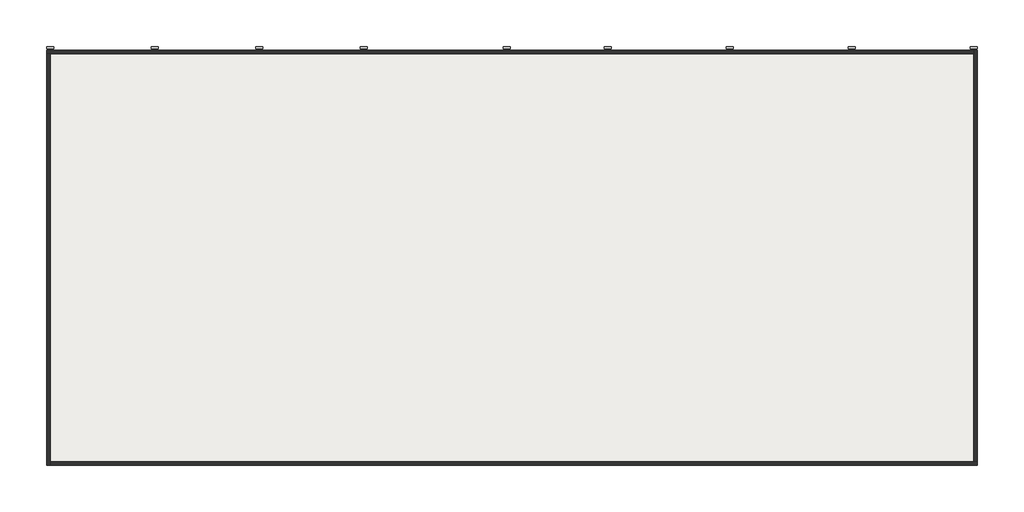
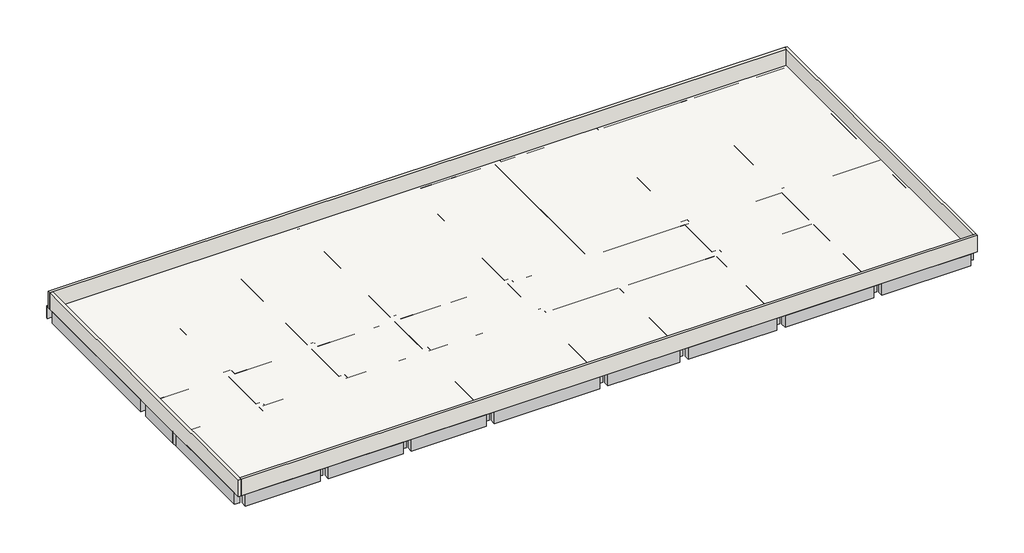
# One storey: 59 beams, 4 walls, 1 slab.
"""IFC4 building model written with IfcOpenShell, lengths in millimetres."""

from ifc_helpers import new_model, si_unit, frame, origin, place, context, project, spatial, polyline, outline, extrude, faceted_brep, element, save

model = new_model("IFC4")

# Units and contexts
model_context = context("Model", 3, world=origin())
ifc_project = project(units=[si_unit("LENGTHUNIT", "METRE", prefix="MILLI")], contexts=[model_context])

# Site, building, storey
site = spatial("IfcSite", under=ifc_project)
building = spatial("IfcBuilding", under=site)
storey = spatial("IfcBuildingStorey", under=building, Name="TOC", Elevation=7650.0)

# Beams
placement = place(None, origin())
element("IfcBeam", 1, ObjectType="RC Beam_Rectangular : H_SB_ACB_B400xH900", at=placement, inside=storey, context=model_context, shape_type="SweptSolid", body=[
    extrude(outline(polyline([(224.7, 12116.5208589), (224.7, 12516.5208589), (5624.7, 12516.5208589), (5624.7, 12116.5208589), (224.7, 12116.5208589)])), frame((0.0, 0.0, 6750.0), z_axis=(0.0, 0.0, 1.0), x_axis=(1.0, 0.0, 0.0)), (0.0, 0.0, 1.0), 900.0),
])
element("IfcBeam", 2, ObjectType="RC Beam_Rectangular : H_SB_ACB_B400xH900", at=placement, inside=storey, context=model_context, shape_type="SweptSolid", body=[
    extrude(outline(polyline([(6224.7, 12116.5208589), (6224.7, 12516.5208589), (11624.7, 12516.5208589), (11624.7, 12116.5208589), (6224.7, 12116.5208589)])), frame((0.0, 0.0, 6750.0), z_axis=(0.0, 0.0, 1.0), x_axis=(1.0, 0.0, 0.0)), (0.0, 0.0, 1.0), 900.0),
])
element("IfcBeam", 3, ObjectType="RC Beam_Rectangular : H_SB_ACB_B400xH900", at=placement, inside=storey, context=model_context, shape_type="SweptSolid", body=[
    extrude(outline(polyline([(12224.7, 12116.5208589), (12224.7, 12516.5208589), (17624.7, 12516.5208589), (17624.7, 12116.5208589), (12224.7, 12116.5208589)])), frame((0.0, 0.0, 6750.0), z_axis=(0.0, 0.0, 1.0), x_axis=(1.0, 0.0, 0.0)), (0.0, 0.0, 1.0), 900.0),
])
element("IfcBeam", 4, ObjectType="RC Beam_Rectangular : H_SB_ACB_B400xH900", at=placement, inside=storey, context=model_context, shape_type="Brep", body=[
    faceted_brep([(26324.7, 12116.5208589, 7650.0), (26324.7, 12516.5208589, 7650.0), (25924.7, 12516.5208589, 7650.0), (18224.7, 12516.5208589, 7650.0), (18224.7, 12116.5208589, 7650.0), (25924.7, 12116.5208589, 7650.0), (26324.7, 12116.5208589, 6750.0), (18224.7, 12116.5208589, 6750.0), (25924.7, 12116.5208589, 6750.0), (26324.7, 12516.5208589, 6750.0), (18224.7, 12516.5208589, 6750.0), (25924.7, 12516.5208589, 6750.0)], [[[0, 1, 2, 3, 4, 5]], [[6, 0, 5, 4, 7, 8]], [[9, 6, 8, 7, 10, 11]], [[1, 9, 11, 10, 3, 2]], [[4, 3, 10, 7]], [[1, 0, 6, 9]]]),
])
element("IfcBeam", 5, ObjectType="RC Beam_Rectangular : H_SB_ACB_B400xH900", at=placement, inside=storey, context=model_context, shape_type="Brep", body=[
    faceted_brep([(32124.7, 12116.5208589, 7650.0), (32124.7, 12516.5208589, 7650.0), (31724.7, 12516.5208589, 7650.0), (26324.7, 12516.5208589, 7650.0), (26324.7, 12116.5208589, 7650.0), (31724.7, 12116.5208589, 7650.0), (32124.7, 12116.5208589, 6750.0), (26324.7, 12116.5208589, 6750.0), (31724.7, 12116.5208589, 6750.0), (32124.7, 12516.5208589, 6750.0), (26324.7, 12516.5208589, 6750.0), (31724.7, 12516.5208589, 6750.0)], [[[0, 1, 2, 3, 4, 5]], [[6, 0, 5, 4, 7, 8]], [[9, 6, 8, 7, 10, 11]], [[1, 9, 11, 10, 3, 2]], [[1, 0, 6, 9]], [[4, 3, 10, 7]]]),
])
element("IfcBeam", 6, ObjectType="RC Beam_Rectangular : H_SB_ACB_B400xH900", at=placement, inside=storey, context=model_context, shape_type="Brep", body=[
    faceted_brep([(39124.7, 12116.5208589, 7650.0), (39124.7, 12516.5208589, 7650.0), (38724.7, 12516.5208589, 7650.0), (32124.7, 12516.5208589, 7650.0), (32124.7, 12116.5208589, 7650.0), (38724.7, 12116.5208589, 7650.0), (39124.7, 12116.5208589, 6750.0), (32124.7, 12116.5208589, 6750.0), (38724.7, 12116.5208589, 6750.0), (39124.7, 12516.5208589, 6750.0), (32124.7, 12516.5208589, 6750.0), (38724.7, 12516.5208589, 6750.0)], [[[0, 1, 2, 3, 4, 5]], [[6, 0, 5, 4, 7, 8]], [[9, 6, 8, 7, 10, 11]], [[1, 9, 11, 10, 3, 2]], [[1, 0, 6, 9]], [[4, 3, 10, 7]]]),
])
element("IfcBeam", 7, ObjectType="RC Beam_Rectangular : H_SB_ACB_B400xH900", at=placement, inside=storey, context=model_context, shape_type="Brep", body=[
    faceted_brep([(46124.7, 12116.5208589, 7650.0), (46124.7, 12516.5208589, 7650.0), (45724.7, 12516.5208589, 7650.0), (39124.7, 12516.5208589, 7650.0), (39124.7, 12116.5208589, 7650.0), (45724.7, 12116.5208589, 7650.0), (46124.7, 12116.5208589, 6750.0), (39124.7, 12116.5208589, 6750.0), (45724.7, 12116.5208589, 6750.0), (46124.7, 12516.5208589, 6750.0), (39124.7, 12516.5208589, 6750.0), (45724.7, 12516.5208589, 6750.0)], [[[0, 1, 2, 3, 4, 5]], [[6, 0, 5, 4, 7, 8]], [[9, 6, 8, 7, 10, 11]], [[1, 9, 11, 10, 3, 2]], [[1, 0, 6, 9]], [[4, 3, 10, 7]]]),
])
element("IfcBeam", 8, ObjectType="RC Beam_Rectangular : H_SB_ACB_B400xH900", at=placement, inside=storey, context=model_context, shape_type="Brep", body=[
    faceted_brep([(53124.7, 12116.5208589, 7650.0), (53124.7, 12516.5208589, 7650.0), (52724.7, 12516.5208589, 7650.0), (46124.7, 12516.5208589, 7650.0), (46124.7, 12116.5208589, 7650.0), (52724.7, 12116.5208589, 7650.0), (53124.7, 12116.5208589, 6750.0), (46124.7, 12116.5208589, 6750.0), (52724.7, 12116.5208589, 6750.0), (53124.7, 12516.5208589, 6750.0), (46124.7, 12516.5208589, 6750.0), (52724.7, 12516.5208589, 6750.0)], [[[0, 1, 2, 3, 4, 5]], [[6, 0, 5, 4, 7, 8]], [[9, 6, 8, 7, 10, 11]], [[1, 9, 11, 10, 3, 2]], [[1, 0, 6, 9]], [[4, 3, 10, 7]]]),
])
element("IfcBeam", 9, ObjectType="RC Beam_Rectangular : H_SB_ACB_B400xH900", at=placement, inside=storey, context=model_context, shape_type="SweptSolid", body=[
    extrude(outline(polyline([(224.7, 23816.5208589), (224.7, 24216.5208589), (5624.7, 24216.5208589), (5624.7, 23816.5208589), (224.7, 23816.5208589)])), frame((0.0, 0.0, 6750.0), z_axis=(0.0, 0.0, 1.0), x_axis=(1.0, 0.0, 0.0)), (0.0, 0.0, 1.0), 900.0),
])
element("IfcBeam", 10, ObjectType="RC Beam_Rectangular : H_SB_ACB_B400xH900", at=placement, inside=storey, context=model_context, shape_type="SweptSolid", body=[
    extrude(outline(polyline([(6224.7, 23816.5208589), (6224.7, 24216.5208589), (11624.7, 24216.5208589), (11624.7, 23816.5208589), (6224.7, 23816.5208589)])), frame((0.0, 0.0, 6750.0), z_axis=(0.0, 0.0, 1.0), x_axis=(1.0, 0.0, 0.0)), (0.0, 0.0, 1.0), 900.0),
])
element("IfcBeam", 11, ObjectType="RC Beam_Rectangular : H_SB_ACB_B400xH900", at=placement, inside=storey, context=model_context, shape_type="SweptSolid", body=[
    extrude(outline(polyline([(12224.7, 23816.5208589), (12224.7, 24216.5208589), (17624.7, 24216.5208589), (17624.7, 23816.5208589), (12224.7, 23816.5208589)])), frame((0.0, 0.0, 6750.0), z_axis=(0.0, 0.0, 1.0), x_axis=(1.0, 0.0, 0.0)), (0.0, 0.0, 1.0), 900.0),
])
element("IfcBeam", 12, ObjectType="RC Beam_Rectangular : H_SB_ACB_B400xH900", at=placement, inside=storey, context=model_context, shape_type="SweptSolid", body=[
    extrude(outline(polyline([(18224.7, 23816.5208589), (18224.7, 24216.5208589), (25824.7, 24216.5208589), (25824.7, 23816.5208589), (18224.7, 23816.5208589)])), frame((0.0, 0.0, 6750.0), z_axis=(0.0, 0.0, 1.0), x_axis=(1.0, 0.0, 0.0)), (0.0, 0.0, 1.0), 900.0),
])
element("IfcBeam", 13, ObjectType="RC Beam_Rectangular : H_SB_ACB_B400xH900", at=placement, inside=storey, context=model_context, shape_type="SweptSolid", body=[
    extrude(outline(polyline([(26424.7, 23816.5208589), (26424.7, 24216.5208589), (31624.7, 24216.5208589), (31624.7, 23816.5208589), (26424.7, 23816.5208589)])), frame((0.0, 0.0, 6750.0), z_axis=(0.0, 0.0, 1.0), x_axis=(1.0, 0.0, 0.0)), (0.0, 0.0, 1.0), 900.0),
])
element("IfcBeam", 14, ObjectType="RC Beam_Rectangular : H_SB_ACB_B400xH900", at=placement, inside=storey, context=model_context, shape_type="SweptSolid", body=[
    extrude(outline(polyline([(32224.7, 23816.5208589), (32224.7, 24216.5208589), (38624.7, 24216.5208589), (38624.7, 23816.5208589), (32224.7, 23816.5208589)])), frame((0.0, 0.0, 6750.0), z_axis=(0.0, 0.0, 1.0), x_axis=(1.0, 0.0, 0.0)), (0.0, 0.0, 1.0), 900.0),
])
element("IfcBeam", 15, ObjectType="RC Beam_Rectangular : H_SB_ACB_B400xH900", at=placement, inside=storey, context=model_context, shape_type="SweptSolid", body=[
    extrude(outline(polyline([(39224.7, 23816.5208589), (39224.7, 24216.5208589), (45624.7, 24216.5208589), (45624.7, 23816.5208589), (39224.7, 23816.5208589)])), frame((0.0, 0.0, 6750.0), z_axis=(0.0, 0.0, 1.0), x_axis=(1.0, 0.0, 0.0)), (0.0, 0.0, 1.0), 900.0),
])
element("IfcBeam", 16, ObjectType="RC Beam_Rectangular : H_SB_ACB_B400xH900", at=placement, inside=storey, context=model_context, shape_type="SweptSolid", body=[
    extrude(outline(polyline([(46224.7, 23816.5208589), (46224.7, 24216.5208589), (52624.7, 24216.5208589), (52624.7, 23816.5208589), (46224.7, 23816.5208589)])), frame((0.0, 0.0, 6750.0), z_axis=(0.0, 0.0, 1.0), x_axis=(1.0, 0.0, 0.0)), (0.0, 0.0, 1.0), 900.0),
])
element("IfcBeam", 17, ObjectType="RC Beam_Rectangular : H_SB_ACB_B400xH900", at=placement, inside=storey, context=model_context, shape_type="Brep", body=[
    faceted_brep([(-275.3, 8616.5208589, 7650.0), (-275.3, 8216.5208589, 7650.0), (124.7, 8216.5208589, 7650.0), (5724.7, 8216.5208589, 7650.0), (6124.7, 8216.5208589, 7650.0), (6124.7, 8616.5208589, 7650.0), (5724.7, 8616.5208589, 7650.0), (124.7, 8616.5208589, 7650.0), (-275.3, 8216.5208589, 6750.0), (124.7, 8216.5208589, 6750.0), (5724.7, 8216.5208589, 6750.0), (6124.7, 8216.5208589, 6750.0), (-275.3, 8616.5208589, 6750.0), (124.7, 8616.5208589, 6750.0), (5724.7, 8616.5208589, 6750.0), (6124.7, 8616.5208589, 6750.0)], [[[0, 1, 2, 3, 4, 5, 6, 7]], [[1, 8, 9, 10, 11, 4, 3, 2]], [[8, 12, 13, 14, 15, 11, 10, 9]], [[12, 0, 7, 6, 5, 15, 14, 13]], [[1, 0, 12, 8]], [[5, 4, 11, 15]]]),
])
element("IfcBeam", 18, ObjectType="RC Beam_Rectangular : H_SB_ACB_B400xH900", at=placement, inside=storey, context=model_context, shape_type="Brep", body=[
    faceted_brep([(12124.7, 8216.5208589, 7650.0), (12124.7, 8616.5208589, 7650.0), (11724.7, 8616.5208589, 7650.0), (6124.7, 8616.5208589, 7650.0), (6124.7, 8216.5208589, 7650.0), (11724.7, 8216.5208589, 7650.0), (12124.7, 8216.5208589, 6750.0), (6124.7, 8216.5208589, 6750.0), (11724.7, 8216.5208589, 6750.0), (12124.7, 8616.5208589, 6750.0), (6124.7, 8616.5208589, 6750.0), (11724.7, 8616.5208589, 6750.0)], [[[0, 1, 2, 3, 4, 5]], [[6, 0, 5, 4, 7, 8]], [[9, 6, 8, 7, 10, 11]], [[1, 9, 11, 10, 3, 2]], [[1, 0, 6, 9]], [[4, 3, 10, 7]]]),
])
element("IfcBeam", 19, ObjectType="RC Beam_Rectangular : H_SB_ACB_B400xH900", at=placement, inside=storey, context=model_context, shape_type="Brep", body=[
    faceted_brep([(18124.7, 8216.5208589, 7650.0), (18124.7, 8616.5208589, 7650.0), (17724.7, 8616.5208589, 7650.0), (12124.7, 8616.5208589, 7650.0), (12124.7, 8216.5208589, 7650.0), (17724.7, 8216.5208589, 7650.0), (18124.7, 8216.5208589, 6750.0), (12124.7, 8216.5208589, 6750.0), (17724.7, 8216.5208589, 6750.0), (18124.7, 8616.5208589, 6750.0), (12124.7, 8616.5208589, 6750.0), (17724.7, 8616.5208589, 6750.0)], [[[0, 1, 2, 3, 4, 5]], [[6, 0, 5, 4, 7, 8]], [[9, 6, 8, 7, 10, 11]], [[1, 9, 11, 10, 3, 2]], [[1, 0, 6, 9]], [[4, 3, 10, 7]]]),
])
element("IfcBeam", 20, ObjectType="RC Beam_Rectangular : H_SB_ACB_B400xH900", at=placement, inside=storey, context=model_context, shape_type="SweptSolid", body=[
    extrude(outline(polyline([(18124.7, 8216.5208589), (18124.7, 8616.5208589), (25824.7, 8616.5208589), (25824.7, 8216.5208589), (18124.7, 8216.5208589)])), frame((0.0, 0.0, 6750.0), z_axis=(0.0, 0.0, 1.0), x_axis=(1.0, 0.0, 0.0)), (0.0, 0.0, 1.0), 900.0),
])
element("IfcBeam", 21, ObjectType="RC Beam_Rectangular : H_SB_ACB_B400xH900", at=placement, inside=storey, context=model_context, shape_type="SweptSolid", body=[
    extrude(outline(polyline([(26424.7, 8216.5208589), (26424.7, 8616.5208589), (31624.7, 8616.5208589), (31624.7, 8216.5208589), (26424.7, 8216.5208589)])), frame((0.0, 0.0, 6750.0), z_axis=(0.0, 0.0, 1.0), x_axis=(1.0, 0.0, 0.0)), (0.0, 0.0, 1.0), 900.0),
])
element("IfcBeam", 22, ObjectType="RC Beam_Rectangular : H_SB_ACB_B400xH900", at=placement, inside=storey, context=model_context, shape_type="SweptSolid", body=[
    extrude(outline(polyline([(32224.7, 8216.5208589), (32224.7, 8616.5208589), (38624.7, 8616.5208589), (38624.7, 8216.5208589), (32224.7, 8216.5208589)])), frame((0.0, 0.0, 6750.0), z_axis=(0.0, 0.0, 1.0), x_axis=(1.0, 0.0, 0.0)), (0.0, 0.0, 1.0), 900.0),
])
element("IfcBeam", 23, ObjectType="RC Beam_Rectangular : H_SB_ACB_B400xH900", at=placement, inside=storey, context=model_context, shape_type="SweptSolid", body=[
    extrude(outline(polyline([(39224.7, 8216.5208589), (39224.7, 8616.5208589), (45624.7, 8616.5208589), (45624.7, 8216.5208589), (39224.7, 8216.5208589)])), frame((0.0, 0.0, 6750.0), z_axis=(0.0, 0.0, 1.0), x_axis=(1.0, 0.0, 0.0)), (0.0, 0.0, 1.0), 900.0),
])
element("IfcBeam", 24, ObjectType="RC Beam_Rectangular : H_SB_ACB_B400xH900", at=placement, inside=storey, context=model_context, shape_type="SweptSolid", body=[
    extrude(outline(polyline([(46224.7, 8216.5208589), (46224.7, 8616.5208589), (52624.7, 8616.5208589), (52624.7, 8216.5208589), (46224.7, 8216.5208589)])), frame((0.0, 0.0, 6750.0), z_axis=(0.0, 0.0, 1.0), x_axis=(1.0, 0.0, 0.0)), (0.0, 0.0, 1.0), 900.0),
])
element("IfcBeam", 25, ObjectType="RC Beam_Rectangular : H_SB_ACB_B400xH900", at=placement, inside=storey, context=model_context, shape_type="SweptSolid", body=[
    extrude(outline(polyline([(224.7, 416.5208589), (224.7, 816.5208589), (5624.7, 816.5208589), (5624.7, 416.5208589), (224.7, 416.5208589)])), frame((0.0, 0.0, 6750.0), z_axis=(0.0, 0.0, 1.0), x_axis=(1.0, 0.0, 0.0)), (0.0, 0.0, 1.0), 900.0),
])
element("IfcBeam", 26, ObjectType="RC Beam_Rectangular : H_SB_ACB_B400xH900", at=placement, inside=storey, context=model_context, shape_type="SweptSolid", body=[
    extrude(outline(polyline([(6224.7, 416.5208589), (6224.7, 816.5208589), (11624.7, 816.5208589), (11624.7, 416.5208589), (6224.7, 416.5208589)])), frame((0.0, 0.0, 6750.0), z_axis=(0.0, 0.0, 1.0), x_axis=(1.0, 0.0, 0.0)), (0.0, 0.0, 1.0), 900.0),
])
element("IfcBeam", 27, ObjectType="RC Beam_Rectangular : H_SB_ACB_B400xH900", at=placement, inside=storey, context=model_context, shape_type="SweptSolid", body=[
    extrude(outline(polyline([(12224.7, 416.5208589), (12224.7, 816.5208589), (17624.7, 816.5208589), (17624.7, 416.5208589), (12224.7, 416.5208589)])), frame((0.0, 0.0, 6750.0), z_axis=(0.0, 0.0, 1.0), x_axis=(1.0, 0.0, 0.0)), (0.0, 0.0, 1.0), 900.0),
])
element("IfcBeam", 28, ObjectType="RC Beam_Rectangular : H_SB_ACB_B400xH900", at=placement, inside=storey, context=model_context, shape_type="SweptSolid", body=[
    extrude(outline(polyline([(18224.7, 416.5208589), (18224.7, 816.5208589), (25824.7, 816.5208589), (25824.7, 416.5208589), (18224.7, 416.5208589)])), frame((0.0, 0.0, 6750.0), z_axis=(0.0, 0.0, 1.0), x_axis=(1.0, 0.0, 0.0)), (0.0, 0.0, 1.0), 900.0),
])
element("IfcBeam", 29, ObjectType="RC Beam_Rectangular : H_SB_ACB_B400xH900", at=placement, inside=storey, context=model_context, shape_type="SweptSolid", body=[
    extrude(outline(polyline([(26424.7, 416.5208589), (26424.7, 816.5208589), (31624.7, 816.5208589), (31624.7, 416.5208589), (26424.7, 416.5208589)])), frame((0.0, 0.0, 6750.0), z_axis=(0.0, 0.0, 1.0), x_axis=(1.0, 0.0, 0.0)), (0.0, 0.0, 1.0), 900.0),
])
element("IfcBeam", 30, ObjectType="RC Beam_Rectangular : H_SB_ACB_B400xH900", at=placement, inside=storey, context=model_context, shape_type="SweptSolid", body=[
    extrude(outline(polyline([(32224.7, 416.5208589), (32224.7, 816.5208589), (38624.7, 816.5208589), (38624.7, 416.5208589), (32224.7, 416.5208589)])), frame((0.0, 0.0, 6750.0), z_axis=(0.0, 0.0, 1.0), x_axis=(1.0, 0.0, 0.0)), (0.0, 0.0, 1.0), 900.0),
])
element("IfcBeam", 31, ObjectType="RC Beam_Rectangular : H_SB_ACB_B400xH900", at=placement, inside=storey, context=model_context, shape_type="SweptSolid", body=[
    extrude(outline(polyline([(39224.7, 416.5208589), (39224.7, 816.5208589), (45624.7, 816.5208589), (45624.7, 416.5208589), (39224.7, 416.5208589)])), frame((0.0, 0.0, 6750.0), z_axis=(0.0, 0.0, 1.0), x_axis=(1.0, 0.0, 0.0)), (0.0, 0.0, 1.0), 900.0),
])
element("IfcBeam", 32, ObjectType="RC Beam_Rectangular : H_SB_ACB_B400xH900", at=placement, inside=storey, context=model_context, shape_type="SweptSolid", body=[
    extrude(outline(polyline([(46224.7, 416.5208589), (46224.7, 816.5208589), (52624.7, 816.5208589), (52624.7, 416.5208589), (46224.7, 416.5208589)])), frame((0.0, 0.0, 6750.0), z_axis=(0.0, 0.0, 1.0), x_axis=(1.0, 0.0, 0.0)), (0.0, 0.0, 1.0), 900.0),
])
element("IfcBeam", 33, ObjectType="RC Beam_Rectangular : H_SB_ACB_B400xH900", at=placement, inside=storey, context=model_context, shape_type="SweptSolid", body=[
    extrude(outline(polyline([(-275.3, 8216.5208589), (124.7, 8216.5208589), (124.7, 916.5208589), (-275.3, 916.5208589), (-275.3, 8216.5208589)])), frame((0.0, 0.0, 6750.0), z_axis=(0.0, 0.0, 1.0), x_axis=(1.0, 0.0, 0.0)), (0.0, 0.0, 1.0), 900.0),
])
element("IfcBeam", 34, ObjectType="RC Beam_Rectangular : H_SB_ACB_B400xH900", at=placement, inside=storey, context=model_context, shape_type="SweptSolid", body=[
    extrude(outline(polyline([(124.7, 8616.5208589), (-275.3, 8616.5208589), (-275.3, 12016.5208589), (124.7, 12016.5208589), (124.7, 8616.5208589)])), frame((0.0, 0.0, 6750.0), z_axis=(0.0, 0.0, 1.0), x_axis=(1.0, 0.0, 0.0)), (0.0, 0.0, 1.0), 900.0),
])
element("IfcBeam", 35, ObjectType="RC Beam_Rectangular : H_SB_ACB_B400xH900", at=placement, inside=storey, context=model_context, shape_type="SweptSolid", body=[
    extrude(outline(polyline([(-275.3, 24429.2208589), (124.7, 24429.2208589), (124.7, 24316.5208589), (-275.3, 24316.5208589), (-275.3, 24429.2208589)])), frame((0.0, 0.0, 6750.0), z_axis=(0.0, 0.0, 1.0), x_axis=(1.0, 0.0, 0.0)), (0.0, 0.0, 1.0), 900.0),
    extrude(outline(polyline([(124.7, 12616.5208589), (-275.3, 12616.5208589), (-275.3, 23716.5208589), (124.7, 23716.5208589), (124.7, 12616.5208589)])), frame((0.0, 0.0, 6750.0), z_axis=(0.0, 0.0, 1.0), x_axis=(1.0, 0.0, 0.0)), (0.0, 0.0, 1.0), 900.0),
])
element("IfcBeam", 36, ObjectType="RC Beam_Rectangular : H_SB_ACB_B400xH900", at=placement, inside=storey, context=model_context, shape_type="SweptSolid", body=[
    extrude(outline(polyline([(5724.7, 8216.5208589), (6124.7, 8216.5208589), (6124.7, 916.5208589), (5724.7, 916.5208589), (5724.7, 8216.5208589)])), frame((0.0, 0.0, 6750.0), z_axis=(0.0, 0.0, 1.0), x_axis=(1.0, 0.0, 0.0)), (0.0, 0.0, 1.0), 900.0),
])
element("IfcBeam", 37, ObjectType="RC Beam_Rectangular : H_SB_ACB_B400xH900", at=placement, inside=storey, context=model_context, shape_type="SweptSolid", body=[
    extrude(outline(polyline([(6124.7, 8616.5208589), (5724.7, 8616.5208589), (5724.7, 12016.5208589), (6124.7, 12016.5208589), (6124.7, 8616.5208589)])), frame((0.0, 0.0, 6750.0), z_axis=(0.0, 0.0, 1.0), x_axis=(1.0, 0.0, 0.0)), (0.0, 0.0, 1.0), 900.0),
])
element("IfcBeam", 38, ObjectType="RC Beam_Rectangular : H_SB_ACB_B400xH900", at=placement, inside=storey, context=model_context, shape_type="SweptSolid", body=[
    extrude(outline(polyline([(5724.7, 24429.2208589), (6124.7, 24429.2208589), (6124.7, 24316.5208589), (5724.7, 24316.5208589), (5724.7, 24429.2208589)])), frame((0.0, 0.0, 6750.0), z_axis=(0.0, 0.0, 1.0), x_axis=(1.0, 0.0, 0.0)), (0.0, 0.0, 1.0), 900.0),
    extrude(outline(polyline([(6124.7, 12616.5208589), (5724.7, 12616.5208589), (5724.7, 23716.5208589), (6124.7, 23716.5208589), (6124.7, 12616.5208589)])), frame((0.0, 0.0, 6750.0), z_axis=(0.0, 0.0, 1.0), x_axis=(1.0, 0.0, 0.0)), (0.0, 0.0, 1.0), 900.0),
])
element("IfcBeam", 39, ObjectType="RC Beam_Rectangular : H_SB_ACB_B400xH900", at=placement, inside=storey, context=model_context, shape_type="SweptSolid", body=[
    extrude(outline(polyline([(11724.7, 8216.5208589), (12124.7, 8216.5208589), (12124.7, 916.5208589), (11724.7, 916.5208589), (11724.7, 8216.5208589)])), frame((0.0, 0.0, 6750.0), z_axis=(0.0, 0.0, 1.0), x_axis=(1.0, 0.0, 0.0)), (0.0, 0.0, 1.0), 900.0),
])
element("IfcBeam", 40, ObjectType="RC Beam_Rectangular : H_SB_ACB_B400xH900", at=placement, inside=storey, context=model_context, shape_type="SweptSolid", body=[
    extrude(outline(polyline([(12124.7, 8616.5208589), (11724.7, 8616.5208589), (11724.7, 12016.5208589), (12124.7, 12016.5208589), (12124.7, 8616.5208589)])), frame((0.0, 0.0, 6750.0), z_axis=(0.0, 0.0, 1.0), x_axis=(1.0, 0.0, 0.0)), (0.0, 0.0, 1.0), 900.0),
])
element("IfcBeam", 41, ObjectType="RC Beam_Rectangular : H_SB_ACB_B400xH900", at=placement, inside=storey, context=model_context, shape_type="SweptSolid", body=[
    extrude(outline(polyline([(11724.7, 24429.2208589), (12124.7, 24429.2208589), (12124.7, 24316.5208589), (11724.7, 24316.5208589), (11724.7, 24429.2208589)])), frame((0.0, 0.0, 6750.0), z_axis=(0.0, 0.0, 1.0), x_axis=(1.0, 0.0, 0.0)), (0.0, 0.0, 1.0), 900.0),
    extrude(outline(polyline([(12124.7, 12616.5208589), (11724.7, 12616.5208589), (11724.7, 23716.5208589), (12124.7, 23716.5208589), (12124.7, 12616.5208589)])), frame((0.0, 0.0, 6750.0), z_axis=(0.0, 0.0, 1.0), x_axis=(1.0, 0.0, 0.0)), (0.0, 0.0, 1.0), 900.0),
])
element("IfcBeam", 42, ObjectType="RC Beam_Rectangular : H_SB_ACB_B400xH900", at=placement, inside=storey, context=model_context, shape_type="SweptSolid", body=[
    extrude(outline(polyline([(17724.7, 8216.5208589), (18124.7, 8216.5208589), (18124.7, 916.5208589), (17724.7, 916.5208589), (17724.7, 8216.5208589)])), frame((0.0, 0.0, 6750.0), z_axis=(0.0, 0.0, 1.0), x_axis=(1.0, 0.0, 0.0)), (0.0, 0.0, 1.0), 900.0),
])
element("IfcBeam", 43, ObjectType="RC Beam_Rectangular : H_SB_ACB_B400xH900", at=placement, inside=storey, context=model_context, shape_type="SweptSolid", body=[
    extrude(outline(polyline([(18124.7, 8616.5208589), (17724.7, 8616.5208589), (17724.7, 12016.5208589), (18124.7, 12016.5208589), (18124.7, 8616.5208589)])), frame((0.0, 0.0, 6750.0), z_axis=(0.0, 0.0, 1.0), x_axis=(1.0, 0.0, 0.0)), (0.0, 0.0, 1.0), 900.0),
])
element("IfcBeam", 44, ObjectType="RC Beam_Rectangular : H_SB_ACB_B400xH900", at=placement, inside=storey, context=model_context, shape_type="SweptSolid", body=[
    extrude(outline(polyline([(17724.7, 24429.2208589), (18124.7, 24429.2208589), (18124.7, 24316.5208589), (17724.7, 24316.5208589), (17724.7, 24429.2208589)])), frame((0.0, 0.0, 6750.0), z_axis=(0.0, 0.0, 1.0), x_axis=(1.0, 0.0, 0.0)), (0.0, 0.0, 1.0), 900.0),
    extrude(outline(polyline([(18124.7, 12616.5208589), (17724.7, 12616.5208589), (17724.7, 23716.5208589), (18124.7, 23716.5208589), (18124.7, 12616.5208589)])), frame((0.0, 0.0, 6750.0), z_axis=(0.0, 0.0, 1.0), x_axis=(1.0, 0.0, 0.0)), (0.0, 0.0, 1.0), 900.0),
])
element("IfcBeam", 45, ObjectType="RC Beam_Rectangular : H_SB_ACB_B400xH900", at=placement, inside=storey, context=model_context, shape_type="SweptSolid", body=[
    extrude(outline(polyline([(25924.7, 8116.5208589), (26324.7, 8116.5208589), (26324.7, 916.5208589), (25924.7, 916.5208589), (25924.7, 8116.5208589)])), frame((0.0, 0.0, 6750.0), z_axis=(0.0, 0.0, 1.0), x_axis=(1.0, 0.0, 0.0)), (0.0, 0.0, 1.0), 900.0),
])
element("IfcBeam", 46, ObjectType="RC Beam_Rectangular : H_SB_ACB_B400xH900", at=placement, inside=storey, context=model_context, shape_type="SweptSolid", body=[
    extrude(outline(polyline([(25924.7, 12116.5208589), (26324.7, 12116.5208589), (26324.7, 8716.5208589), (25924.7, 8716.5208589), (25924.7, 12116.5208589)])), frame((0.0, 0.0, 6750.0), z_axis=(0.0, 0.0, 1.0), x_axis=(1.0, 0.0, 0.0)), (0.0, 0.0, 1.0), 900.0),
])
element("IfcBeam", 47, ObjectType="RC Beam_Rectangular : H_SB_ACB_B400xH900", at=placement, inside=storey, context=model_context, shape_type="SweptSolid", body=[
    extrude(outline(polyline([(25924.7, 24429.2208589), (26324.7, 24429.2208589), (26324.7, 24316.5208589), (25924.7, 24316.5208589), (25924.7, 24429.2208589)])), frame((0.0, 0.0, 6750.0), z_axis=(0.0, 0.0, 1.0), x_axis=(1.0, 0.0, 0.0)), (0.0, 0.0, 1.0), 900.0),
    extrude(outline(polyline([(26324.7, 12516.5208589), (25924.7, 12516.5208589), (25924.7, 23716.5208589), (26324.7, 23716.5208589), (26324.7, 12516.5208589)])), frame((0.0, 0.0, 6750.0), z_axis=(0.0, 0.0, 1.0), x_axis=(1.0, 0.0, 0.0)), (0.0, 0.0, 1.0), 900.0),
])
element("IfcBeam", 48, ObjectType="RC Beam_Rectangular : H_SB_ACB_B400xH900", at=placement, inside=storey, context=model_context, shape_type="SweptSolid", body=[
    extrude(outline(polyline([(31724.7, 8116.5208589), (32124.7, 8116.5208589), (32124.7, 916.5208589), (31724.7, 916.5208589), (31724.7, 8116.5208589)])), frame((0.0, 0.0, 6750.0), z_axis=(0.0, 0.0, 1.0), x_axis=(1.0, 0.0, 0.0)), (0.0, 0.0, 1.0), 900.0),
])
element("IfcBeam", 49, ObjectType="RC Beam_Rectangular : H_SB_ACB_B400xH900", at=placement, inside=storey, context=model_context, shape_type="SweptSolid", body=[
    extrude(outline(polyline([(31724.7, 12116.5208589), (32124.7, 12116.5208589), (32124.7, 8716.5208589), (31724.7, 8716.5208589), (31724.7, 12116.5208589)])), frame((0.0, 0.0, 6750.0), z_axis=(0.0, 0.0, 1.0), x_axis=(1.0, 0.0, 0.0)), (0.0, 0.0, 1.0), 900.0),
])
element("IfcBeam", 50, ObjectType="RC Beam_Rectangular : H_SB_ACB_B400xH900", at=placement, inside=storey, context=model_context, shape_type="SweptSolid", body=[
    extrude(outline(polyline([(31724.7, 24429.2208589), (32124.7, 24429.2208589), (32124.7, 24316.5208589), (31724.7, 24316.5208589), (31724.7, 24429.2208589)])), frame((0.0, 0.0, 6750.0), z_axis=(0.0, 0.0, 1.0), x_axis=(1.0, 0.0, 0.0)), (0.0, 0.0, 1.0), 900.0),
    extrude(outline(polyline([(32124.7, 12516.5208589), (31724.7, 12516.5208589), (31724.7, 23716.5208589), (32124.7, 23716.5208589), (32124.7, 12516.5208589)])), frame((0.0, 0.0, 6750.0), z_axis=(0.0, 0.0, 1.0), x_axis=(1.0, 0.0, 0.0)), (0.0, 0.0, 1.0), 900.0),
])
element("IfcBeam", 51, ObjectType="RC Beam_Rectangular : H_SB_ACB_B400xH900", at=placement, inside=storey, context=model_context, shape_type="SweptSolid", body=[
    extrude(outline(polyline([(38724.7, 8116.5208589), (39124.7, 8116.5208589), (39124.7, 916.5208589), (38724.7, 916.5208589), (38724.7, 8116.5208589)])), frame((0.0, 0.0, 6750.0), z_axis=(0.0, 0.0, 1.0), x_axis=(1.0, 0.0, 0.0)), (0.0, 0.0, 1.0), 900.0),
])
element("IfcBeam", 52, ObjectType="RC Beam_Rectangular : H_SB_ACB_B400xH900", at=placement, inside=storey, context=model_context, shape_type="SweptSolid", body=[
    extrude(outline(polyline([(38724.7, 12116.5208589), (39124.7, 12116.5208589), (39124.7, 8716.5208589), (38724.7, 8716.5208589), (38724.7, 12116.5208589)])), frame((0.0, 0.0, 6750.0), z_axis=(0.0, 0.0, 1.0), x_axis=(1.0, 0.0, 0.0)), (0.0, 0.0, 1.0), 900.0),
])
element("IfcBeam", 53, ObjectType="RC Beam_Rectangular : H_SB_ACB_B400xH900", at=placement, inside=storey, context=model_context, shape_type="SweptSolid", body=[
    extrude(outline(polyline([(38724.7, 24429.2208589), (39124.7, 24429.2208589), (39124.7, 24316.5208589), (38724.7, 24316.5208589), (38724.7, 24429.2208589)])), frame((0.0, 0.0, 6750.0), z_axis=(0.0, 0.0, 1.0), x_axis=(1.0, 0.0, 0.0)), (0.0, 0.0, 1.0), 900.0),
    extrude(outline(polyline([(39124.7, 12516.5208589), (38724.7, 12516.5208589), (38724.7, 23716.5208589), (39124.7, 23716.5208589), (39124.7, 12516.5208589)])), frame((0.0, 0.0, 6750.0), z_axis=(0.0, 0.0, 1.0), x_axis=(1.0, 0.0, 0.0)), (0.0, 0.0, 1.0), 900.0),
])
element("IfcBeam", 54, ObjectType="RC Beam_Rectangular : H_SB_ACB_B400xH900", at=placement, inside=storey, context=model_context, shape_type="SweptSolid", body=[
    extrude(outline(polyline([(45724.7, 8116.5208589), (46124.7, 8116.5208589), (46124.7, 916.5208589), (45724.7, 916.5208589), (45724.7, 8116.5208589)])), frame((0.0, 0.0, 6750.0), z_axis=(0.0, 0.0, 1.0), x_axis=(1.0, 0.0, 0.0)), (0.0, 0.0, 1.0), 900.0),
])
element("IfcBeam", 55, ObjectType="RC Beam_Rectangular : H_SB_ACB_B400xH900", at=placement, inside=storey, context=model_context, shape_type="SweptSolid", body=[
    extrude(outline(polyline([(45724.7, 12116.5208589), (46124.7, 12116.5208589), (46124.7, 8716.5208589), (45724.7, 8716.5208589), (45724.7, 12116.5208589)])), frame((0.0, 0.0, 6750.0), z_axis=(0.0, 0.0, 1.0), x_axis=(1.0, 0.0, 0.0)), (0.0, 0.0, 1.0), 900.0),
])
element("IfcBeam", 56, ObjectType="RC Beam_Rectangular : H_SB_ACB_B400xH900", at=placement, inside=storey, context=model_context, shape_type="SweptSolid", body=[
    extrude(outline(polyline([(45724.7, 24429.2208589), (46124.7, 24429.2208589), (46124.7, 24316.5208589), (45724.7, 24316.5208589), (45724.7, 24429.2208589)])), frame((0.0, 0.0, 6750.0), z_axis=(0.0, 0.0, 1.0), x_axis=(1.0, 0.0, 0.0)), (0.0, 0.0, 1.0), 900.0),
    extrude(outline(polyline([(46124.7, 12516.5208589), (45724.7, 12516.5208589), (45724.7, 23716.5208589), (46124.7, 23716.5208589), (46124.7, 12516.5208589)])), frame((0.0, 0.0, 6750.0), z_axis=(0.0, 0.0, 1.0), x_axis=(1.0, 0.0, 0.0)), (0.0, 0.0, 1.0), 900.0),
])
element("IfcBeam", 57, ObjectType="RC Beam_Rectangular : H_SB_ACB_B400xH900", at=placement, inside=storey, context=model_context, shape_type="SweptSolid", body=[
    extrude(outline(polyline([(52724.7, 8116.5208589), (53124.7, 8116.5208589), (53124.7, 916.5208589), (52724.7, 916.5208589), (52724.7, 8116.5208589)])), frame((0.0, 0.0, 6750.0), z_axis=(0.0, 0.0, 1.0), x_axis=(1.0, 0.0, 0.0)), (0.0, 0.0, 1.0), 900.0),
])
element("IfcBeam", 58, ObjectType="RC Beam_Rectangular : H_SB_ACB_B400xH900", at=placement, inside=storey, context=model_context, shape_type="SweptSolid", body=[
    extrude(outline(polyline([(52724.7, 12116.5208589), (53124.7, 12116.5208589), (53124.7, 8716.5208589), (52724.7, 8716.5208589), (52724.7, 12116.5208589)])), frame((0.0, 0.0, 6750.0), z_axis=(0.0, 0.0, 1.0), x_axis=(1.0, 0.0, 0.0)), (0.0, 0.0, 1.0), 900.0),
])
element("IfcBeam", 59, ObjectType="RC Beam_Rectangular : H_SB_ACB_B400xH900", at=placement, inside=storey, context=model_context, shape_type="SweptSolid", body=[
    extrude(outline(polyline([(52724.7, 24429.2208589), (53124.7, 24429.2208589), (53124.7, 24316.5208589), (52724.7, 24316.5208589), (52724.7, 24429.2208589)])), frame((0.0, 0.0, 6750.0), z_axis=(0.0, 0.0, 1.0), x_axis=(1.0, 0.0, 0.0)), (0.0, 0.0, 1.0), 900.0),
    extrude(outline(polyline([(52724.7, 23716.5208589), (53124.7, 23716.5208589), (53124.7, 12516.5208589), (52724.7, 12516.5208589), (52724.7, 23716.5208589)])), frame((0.0, 0.0, 6750.0), z_axis=(0.0, 0.0, 1.0), x_axis=(1.0, 0.0, 0.0)), (0.0, 0.0, 1.0), 900.0),
])

# Slab
element("IfcSlab", 60, ObjectType="H_FL_AMF_RC Slab_T150", at=placement, inside=storey, context=model_context, shape_type="SweptSolid", body=[
    extrude(outline(polyline([(52924.7, 24016.5208589), (52924.7, 616.5208589), (-75.3, 616.5208589), (-75.3, 24016.5208589), (52924.7, 24016.5208589)])), frame((0.0, 0.0, 7500.0), z_axis=(0.0, 0.0, 1.0), x_axis=(1.0, 0.0, 0.0)), (0.0, 0.0, 1.0), 150.0),
])

# Walls
element("IfcWall", 61, ObjectType="H_WA_AMW_RC Wall_T200 (No Finish)", at=placement, inside=storey, context=model_context, shape_type="Brep", body=[
    faceted_brep([(-275.3, 24016.5208589, 7650.0), (-75.3, 24016.5208589, 7650.0), (52924.7, 24016.5208589, 7650.0), (52924.7, 24016.5208589, 8900.0), (-75.3, 24016.5208589, 8900.0), (-275.3, 24016.5208589, 8900.0), (-275.3, 24216.5208589, 7650.0), (-275.3, 24216.5208589, 8900.0), (52924.7, 24216.5208589, 8900.0), (52924.7, 24216.5208589, 7650.0)], [[[0, 1, 2, 3, 4, 5]], [[6, 7, 8, 9]], [[2, 1, 0, 6, 9]], [[5, 4, 3, 8, 7]], [[0, 5, 7, 6]], [[3, 2, 9, 8]]]),
])
element("IfcWall", 62, ObjectType="H_WA_AMW_RC Wall_T200 (No Finish)", at=placement, inside=storey, context=model_context, shape_type="Brep", body=[
    faceted_brep([(-75.3, 416.5208589, 7650.0), (-75.3, 616.5208589, 7650.0), (-75.3, 24016.5208589, 7650.0), (-75.3, 24016.5208589, 8900.0), (-75.3, 616.5208589, 8900.0), (-75.3, 416.5208589, 8900.0), (-275.3, 416.5208589, 7650.0), (-275.3, 416.5208589, 8900.0), (-275.3, 24016.5208589, 8900.0), (-275.3, 24016.5208589, 7650.0)], [[[0, 1, 2, 3, 4, 5]], [[6, 7, 8, 9]], [[2, 1, 0, 6, 9]], [[5, 4, 3, 8, 7]], [[0, 5, 7, 6]], [[3, 2, 9, 8]]]),
])
element("IfcWall", 63, ObjectType="H_WA_AMW_RC Wall_T200 (No Finish)", at=placement, inside=storey, context=model_context, shape_type="Brep", body=[
    faceted_brep([(53124.7, 616.5208589, 7650.0), (52924.7, 616.5208589, 7650.0), (-75.3, 616.5208589, 7650.0), (-75.3, 616.5208589, 8900.0), (52924.7, 616.5208589, 8900.0), (53124.7, 616.5208589, 8900.0), (53124.7, 416.5208589, 7650.0), (53124.7, 416.5208589, 8900.0), (-75.3, 416.5208589, 8900.0), (-75.3, 416.5208589, 7650.0)], [[[0, 1, 2, 3, 4, 5]], [[6, 7, 8, 9]], [[2, 1, 0, 6, 9]], [[5, 4, 3, 8, 7]], [[0, 5, 7, 6]], [[3, 2, 9, 8]]]),
])
element("IfcWall", 64, ObjectType="H_WA_AMW_RC Wall_T200 (No Finish)", at=placement, inside=storey, context=model_context, shape_type="Brep", body=[
    faceted_brep([(52924.7, 24216.5208589, 7650.0), (52924.7, 24016.5208589, 7650.0), (52924.7, 616.5208589, 7650.0), (52924.7, 616.5208589, 8900.0), (52924.7, 24016.5208589, 8900.0), (52924.7, 24216.5208589, 8900.0), (53124.7, 24216.5208589, 7650.0), (53124.7, 24216.5208589, 8900.0), (53124.7, 616.5208589, 8900.0), (53124.7, 616.5208589, 7650.0)], [[[0, 1, 2, 3, 4, 5]], [[6, 7, 8, 9]], [[2, 1, 0, 6, 9]], [[5, 4, 3, 8, 7]], [[0, 5, 7, 6]], [[3, 2, 9, 8]]]),
])

save(model, "model.ifc")

# Revit data of these elements
# Type "RC Beam_Rectangular : H_SB_ACB_B400xH900"
#   중앙부 하부근 = ""
#   중앙부 상부근 = ""
#   중앙부 보조근 = ""
#   중앙부 늑근 = ""
#   외단부 하부근 = ""
#   외단부 상부근 = ""
#   외단부 보조근 = ""
#   외단부 늑근 = ""
#   부호 = "TG3"
#   내단부 하부근 = ""
#   내단부 상부근 = ""
#   내단부 보조근 = ""
#   내단부 늑근 = ""
#   ALL 하부근 = "3-D20"
#   ALL 상부근 = "3-D20"
#   ALL 보조근 = ""
#   ALL 늑근 = "2-D10 @120"
#   Width = 400.000 mm
#   Height = 900.000 mm
#   Length [instance default] = 1524.000 mm
#   b = 400.000 mm
#   h = 900.000 mm
#   hec_material3 [instance default] = none
#   hec_material2 [instance default] = none
#   hec_material1 [instance default] = none
#   Structural Material [instance default] = none
#   Assembly Code = ""
# Type "H_FL_AMF_RC Slab_T150"
#   Keynote = ""
#   Type Comments = ""
#   Description = ""
#   Function = 1
#   Layers, outside or top first: 150.000 mm no material (function 1)
# Type "H_WA_AMW_RC Wall_T200 (No Finish)"
#   Type Comments = ""
#   Layers, outside or top first: 0.000 mm no material (function 100); 0.000 mm no material (function 100); 200.000 mm no material (function 1); 0.000 mm no material (function 100); 0.000 mm no material (function 100); 0.000 mm no material (function 100)
# Elements 1, 2, 3, 4, 5, 6, 7, 8, 9, 10, 11, 12, 13, 14, 15, 16, 17, 18, 19, 20, 21, 22, 23, 24, 25, 26, 27, 28, 29, 30, 31, 32, 33, 34, 35, 36, 37, 38, 39, 40, 41, 42, 43, 44, 45, 46, 47, 48, 49, 50, 51, 52, 53, 54, 55, 56, 57, 58, 59 (IfcBeam, "RC Beam_Rectangular : H_SB_ACB_B400xH900")
#   hec_material3 = none
#   hec_material2 = none
#   hec_material1 = none
#   Structural Material = none
#   Phase Created = New Construction
# Element 60 (IfcSlab, "H_FL_AMF_RC Slab_T150")
#   Height Offset From Level = 0.000 mm
#   Phase Created = New Construction
#   Materials on its faces: "Default Floor"
# Elements 61, 62, 63, 64 (IfcWall, "H_WA_AMW_RC Wall_T200 (No Finish)")
#   Top Offset = 0.000 mm
#   Base Offset = 0.000 mm
#   wall height = 1250.000 mm
#   Phase Created = New Construction
#   Base Constraint = TOC
#   Top Constraint = TOP
#   Materials on its faces: "Default Wall"
# Materials
#   "Default Floor": class "Miscellaneous", colour RGB 80 80 80, transparency 0
#   "Default Wall": class "Miscellaneous", colour RGB 80 80 80, transparency 0
# Room at (24679.385, 12577.526) mm, phase "New Construction", upper level "TOC", upper offset 2000.000 mm, lower offset 0.000 mm
#   Comments = ""
#   Number = "201"
#   Name = "ROOF"
